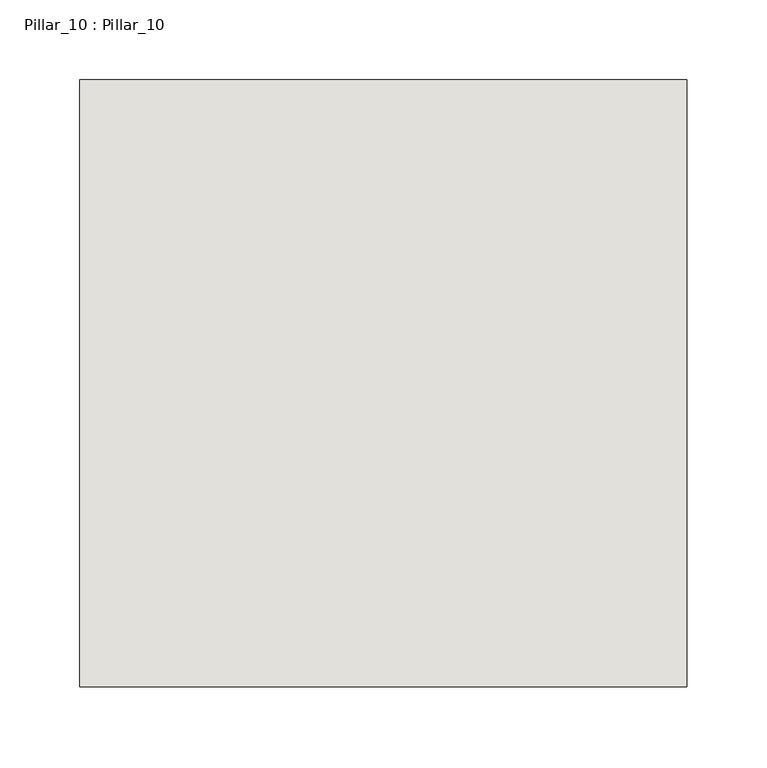
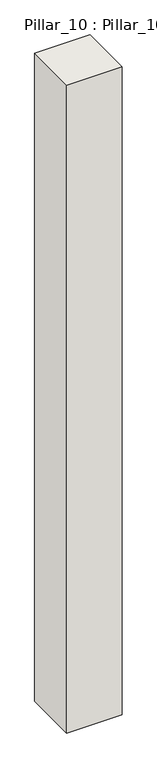
"""IFC4 building model written with IfcOpenShell, lengths in millimetres: wall geometry, Pillar_10 : Pillar_10."""

from ifc_helpers import new_model, si_unit, origin, origin_with_axes, place, context, project, spatial, polyline, outline, extrude, source, transform, mapped, element, save


def pillar_10_pillar_10_9a1170d5(model_context):
    return source(origin(), model_context, "Body", "SweptSolid", [
        extrude(outline(polyline([(5040.0, 0.0), (4660.0, 0.0), (4660.0, 380.0), (5040.0, 380.0), (5040.0, 0.0)])), origin_with_axes(), (0.0, 0.0, 1.0), 4700.0),
    ])


if __name__ == "__main__":
    model = new_model("IFC4")
    model_context = context("Model", 3, world=origin())
    ifc_project = project(units=[si_unit("LENGTHUNIT", "METRE", prefix="MILLI")], contexts=[model_context])
    site = spatial("IfcSite", under=ifc_project)
    building = spatial("IfcBuilding", under=site)
    placement = place(None, origin())
    pillar_10_pillar_10_shape = pillar_10_pillar_10_9a1170d5(model_context)
    element("IfcWall", 1, ObjectType="Pillar_10 : Pillar_10", at=placement, inside=building, context=model_context, shape_type="MappedRepresentation", body=[
        mapped(pillar_10_pillar_10_shape, transform((0.0, 0.0, 0.0), x_axis=(1.0, 0.0, 0.0), y_axis=(0.0, 1.0, 0.0), z_axis=(0.0, 0.0, 1.0))),
    ])
    save(model, "model.ifc")

# Revit data of these elements
# Type "Pillar_10 : Pillar_10"
#   NameOverride = "Pillar_10"
# Element 1 (IfcWall, "Pillar_10 : Pillar_10")
#   Materials on its faces: "IfcSurfaceStyle #33"
# Materials
#   "IfcSurfaceStyle #33": class "Unassigned", colour RGB 214 214 214, transparency 0
